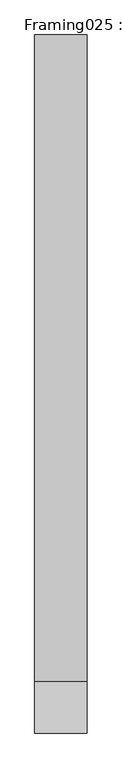
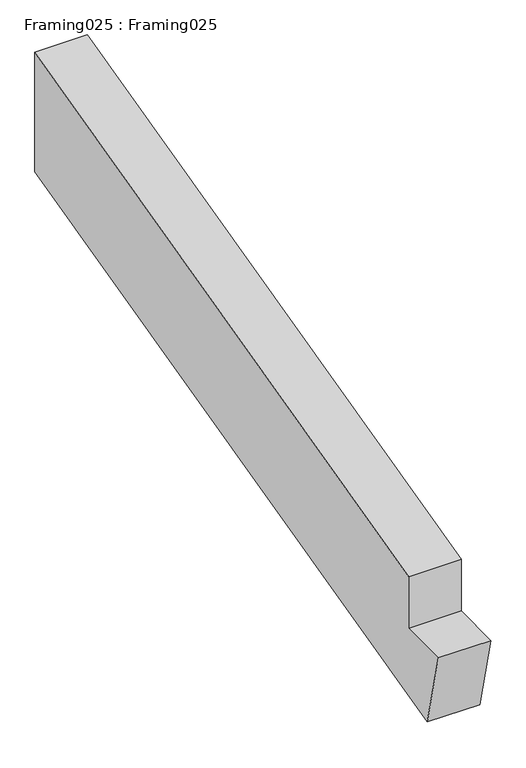
"""IFC4 building model written with IfcOpenShell, lengths in millimetres: proxy geometry, Framing025 : Framing025."""

import ifcopenshell
import ifcopenshell.guid

model = None  # the IFC model being written
_history = None  # IfcOwnerHistory: only IFC2X3 demands one
_inside = {}  # id of a spatial element -> (the spatial element, [elements in it])
_under = {}  # id of a project, library or spatial element -> (it, [spatial elements below it])
_declared = {}  # id of a project -> (the project, [libraries it declares])
_typed = {}  # id of a type object -> (the type object, [elements of that type])
_made_of = {}  # id of a material, layer set ... -> (it, [elements and type objects made of it])


def new_model(schema):
    """Start an empty IFC model of exactly this schema.

    Asked for "IFC4X3", IfcOpenShell would pick the latest addendum, in which some entities
    have other attributes; the version numbers below select the first issue.
    IFC2X3 requires an IfcOwnerHistory on every rooted entity: one is made here for all.
    """
    global model, _history
    if schema == "IFC4X3":
        model = ifcopenshell.file(schema_version=(4, 3, 0, 0))
    else:
        model = ifcopenshell.file(schema=schema)
    _inside.clear()
    _under.clear()
    _declared.clear()
    _typed.clear()
    _made_of.clear()
    _history = None
    if model.schema == "IFC2X3":
        org = make("IfcOrganization", Name="unknown")
        user = make(
            "IfcPersonAndOrganization",
            ThePerson=make("IfcPerson", FamilyName="unknown"),
            TheOrganization=org,
        )
        app = make(
            "IfcApplication",
            ApplicationDeveloper=org,
            Version="unknown",
            ApplicationFullName="unknown",
            ApplicationIdentifier="unknown",
        )
        _history = make(
            "IfcOwnerHistory",
            OwningUser=user,
            OwningApplication=app,
            ChangeAction="ADDED",
            CreationDate=0,
        )
    return model


def make(cls, **values):
    """One entity of the class cls with the attributes given. An attribute that is None is left unset."""
    return model.create_entity(
        cls, **{name: value for name, value in values.items() if value is not None}
    )


def rooted(cls, **values):
    """An entity with a GlobalId (a new one), such as an element, a storey or a relation."""
    return make(cls, GlobalId=ifcopenshell.guid.new(), OwnerHistory=_history, **values)


def si_unit(unit_type, name, prefix=None):
    """IfcSIUnit, for example si_unit("LENGTHUNIT", "METRE", prefix="MILLI")."""
    return make("IfcSIUnit", UnitType=unit_type, Prefix=prefix, Name=name)


def assignment(units):
    """IfcUnitAssignment: the units of a project."""
    return None if units is None else make("IfcUnitAssignment", Units=units)


def point(xyz):
    """IfcCartesianPoint."""
    return None if xyz is None else make("IfcCartesianPoint", Coordinates=xyz)


def direction(xyz):
    """IfcDirection."""
    return None if xyz is None else make("IfcDirection", DirectionRatios=xyz)


def frame(location, z_axis=None, x_axis=None):
    """IfcAxis2Placement3D, a coordinate frame: its origin and axes. An axis left out is left unset."""
    return make(
        "IfcAxis2Placement3D",
        Location=point(location),
        Axis=direction(z_axis),
        RefDirection=direction(x_axis),
    )


def origin():
    """The frame at (0, 0, 0) with its axes left unset."""
    return frame((0.0, 0.0, 0.0))


def place(relative_to, where):
    """IfcLocalPlacement: puts the frame where relative to a parent placement (None: the world)."""
    return make(
        "IfcLocalPlacement", PlacementRelTo=relative_to, RelativePlacement=where
    )


def context(
    kind, dimensions, precision=None, world=None, true_north=None, identifier=None
):
    """IfcGeometricRepresentationContext, for example the 3D "Model" context."""
    return make(
        "IfcGeometricRepresentationContext",
        ContextIdentifier=identifier,
        ContextType=kind,
        CoordinateSpaceDimension=dimensions,
        Precision=precision,
        WorldCoordinateSystem=world,
        TrueNorth=true_north,
    )


def project(units=None, contexts=None):
    """IfcProject with its units and contexts."""
    return rooted(
        "IfcProject",
        Name="project",
        RepresentationContexts=contexts,
        UnitsInContext=assignment(units),
    )


def spatial(cls, under=None, at=None, **own):
    """A site, building, storey or space (cls), placed at a placement, below another one or the project."""
    s = rooted(cls, ObjectPlacement=at, **own)
    if under is not None:
        _under.setdefault(under.id(), (under, []))[1].append(s)
    return s


def polyline(points):
    """IfcPolyline through the points."""
    return make("IfcPolyline", Points=[point(p) for p in points])


def outline(outer, holes=None, kind="AREA"):
    """IfcArbitraryClosedProfileDef: a profile drawn as a closed curve; with holes, ...WithVoids."""
    if holes is None:
        return make("IfcArbitraryClosedProfileDef", ProfileType=kind, OuterCurve=outer)
    return make(
        "IfcArbitraryProfileDefWithVoids",
        ProfileType=kind,
        OuterCurve=outer,
        InnerCurves=holes,
    )


def extrude(swept, where, along, depth):
    """IfcExtrudedAreaSolid: the profile swept, set in the frame where, extruded along a direction by depth."""
    return make(
        "IfcExtrudedAreaSolid",
        SweptArea=swept,
        Position=where,
        ExtrudedDirection=direction(along),
        Depth=depth,
    )


def shape(context_of_items, identifier, shape_type, items):
    """IfcShapeRepresentation: the items that make up one representation, for example the "Body"."""
    return make(
        "IfcShapeRepresentation",
        ContextOfItems=context_of_items,
        RepresentationIdentifier=identifier,
        RepresentationType=shape_type,
        Items=items,
    )


def source(mapping_origin, context_of_items, identifier, shape_type, items):
    """IfcRepresentationMap: a shape defined once, which mapped items show again and again."""
    return make(
        "IfcRepresentationMap",
        MappingOrigin=mapping_origin,
        MappedRepresentation=shape(context_of_items, identifier, shape_type, items),
    )


def transform(
    local_origin,
    x_axis=None,
    y_axis=None,
    z_axis=None,
    scale=None,
    scale2=None,
    scale3=None,
    uniform=True,
):
    """IfcCartesianTransformationOperator3D, or its non-uniform kind. x_axis, y_axis, z_axis: its Axis1, 2, 3."""
    if uniform:
        return make(
            "IfcCartesianTransformationOperator3D",
            Axis1=direction(x_axis),
            Axis2=direction(y_axis),
            LocalOrigin=point(local_origin),
            Scale=scale,
            Axis3=direction(z_axis),
        )
    return make(
        "IfcCartesianTransformationOperator3DnonUniform",
        Axis1=direction(x_axis),
        Axis2=direction(y_axis),
        LocalOrigin=point(local_origin),
        Scale=scale,
        Axis3=direction(z_axis),
        Scale2=scale2,
        Scale3=scale3,
    )


def mapped(mapping_source, mapping_target):
    """IfcMappedItem: shows the shape of a source again, moved by a transform."""
    return make(
        "IfcMappedItem", MappingSource=mapping_source, MappingTarget=mapping_target
    )


def made_of(thing, what):
    """Note that an element or type object is made of a material, layer set ...; save() writes the relation."""
    if what is not None:
        _made_of.setdefault(what.id(), (what, []))[1].append(thing)
    return thing


def element(
    cls,
    number,
    at=None,
    inside=None,
    cuts=None,
    type_object=None,
    material=None,
    context=None,
    identifier="Body",
    shape_type=None,
    held_by="IfcProductDefinitionShape",
    body=None,
    shapes=None,
    **own,
):
    """One element of the class cls, such as IfcWall. Its Tag is "e" and its number.

    at: its placement. inside: the storey or other place that contains it. cuts: it is an
    opening in that element (IfcRelVoidsElement). A single representation is given by context,
    identifier, shape_type and body (its items); several are given by shapes. held_by: the class
    of the entity that holds the representations. save() writes the other relations.
    """
    e = rooted(cls, Tag="e%d" % number, ObjectPlacement=at, **own)
    if body is not None:
        shapes = [shape(context, identifier, shape_type, body)]
    if shapes is not None:
        e.Representation = make(held_by, Representations=shapes)
    if inside is not None:
        _inside.setdefault(inside.id(), (inside, []))[1].append(e)
    if cuts is not None:
        rooted(
            "IfcRelVoidsElement", RelatingBuildingElement=cuts, RelatedOpeningElement=e
        )
    if type_object is not None:
        _typed.setdefault(type_object.id(), (type_object, []))[1].append(e)
    return made_of(e, material)


def aggregate(whole, parts):
    """IfcRelAggregates: a whole, such as a stair, and the parts it consists of."""
    return rooted("IfcRelAggregates", RelatingObject=whole, RelatedObjects=parts)


def save(model, path):
    """Write the relations noted so far, then the file.

    IfcRelAggregates (storeys below a building ...), IfcRelContainedInSpatialStructure (elements
    in a storey), IfcRelDefinesByType, IfcRelAssociatesMaterial and IfcRelDeclares: one each for
    every whole, place, type object, material and project.
    """
    for whole, parts in _under.values():
        aggregate(whole, parts)
    for where, things in _inside.values():
        rooted(
            "IfcRelContainedInSpatialStructure",
            RelatedElements=things,
            RelatingStructure=where,
        )
    for kind, things in _typed.values():
        rooted("IfcRelDefinesByType", RelatedObjects=things, RelatingType=kind)
    for what, things in _made_of.values():
        rooted("IfcRelAssociatesMaterial", RelatedObjects=things, RelatingMaterial=what)
    for by, libraries in _declared.values():
        rooted("IfcRelDeclares", RelatingContext=by, RelatedDefinitions=libraries)
    model.write(path)


def framing025_framing025_fdaa2fb1(model_context):
    return source(origin(), model_context, "Body", "SweptSolid", [
        extrude(outline(polyline([(-5374.9745897, 42642.0307603), (-5224.4076049, 42642.0307603), (-5224.4076049, 42800.8143799), (-3344.6566162, 43270.717426), (-3344.6566162, 42903.8818003), (-5318.455674, 42411.3663805), (-5374.9745897, 42642.0307603)])), frame((12534.9, 0.0, 0.0), z_axis=(1.0, 0.0, 0.0), x_axis=(0.0, 1.0, 0.0)), (0.0, 0.0, 1.0), 152.4),
    ])


if __name__ == "__main__":
    model = new_model("IFC4")
    model_context = context("Model", 3, world=origin())
    ifc_project = project(units=[si_unit("LENGTHUNIT", "METRE", prefix="MILLI")], contexts=[model_context])
    site = spatial("IfcSite", under=ifc_project)
    building = spatial("IfcBuilding", under=site)
    placement = place(None, origin())
    framing025_framing025_shape = framing025_framing025_fdaa2fb1(model_context)
    element("IfcBuildingElementProxy", 1, Name="Framing025 : Framing025", ObjectType="Framing025 : Framing025", at=placement, inside=building, context=model_context, shape_type="MappedRepresentation", body=[
        mapped(framing025_framing025_shape, transform((0.0, 0.0, 0.0), x_axis=(1.0, 0.0, 0.0), y_axis=(0.0, 1.0, 0.0), z_axis=(0.0, 0.0, 1.0))),
    ])
    save(model, "model.ifc")

# Revit data of these elements
# Type "Framing025 : Framing025"
#   NameOverride = "Framing025"
# Element 1 (IfcBuildingElementProxy, "Framing025 : Framing025")
#   Materials on its faces: "WOOD FRAMING (SEE STRUCT DWGS)"
# Materials
#   "WOOD FRAMING (SEE STRUCT DWGS)": class "Unassigned", colour RGB 224 188 168, transparency 0, Cost = 0
